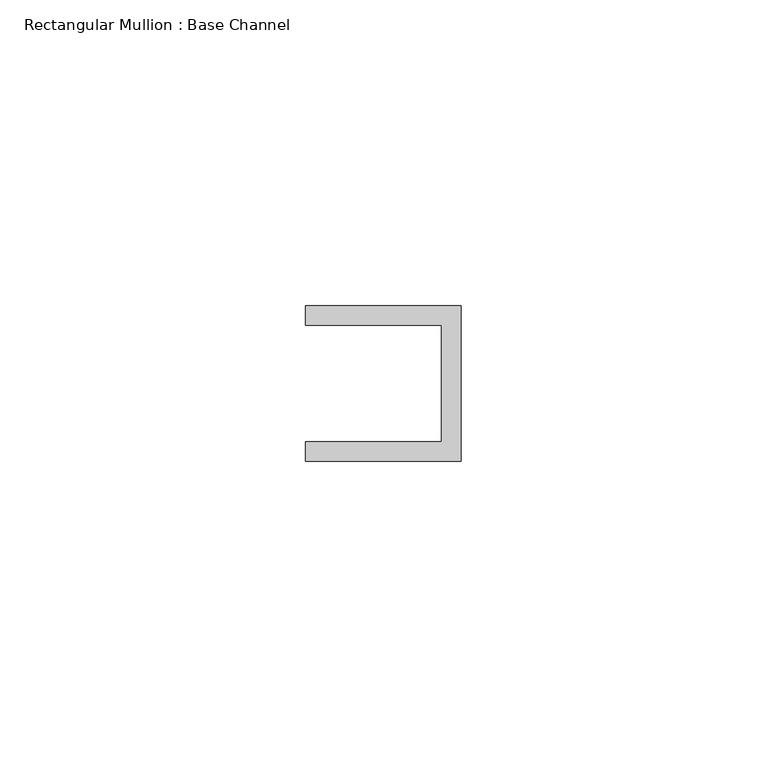
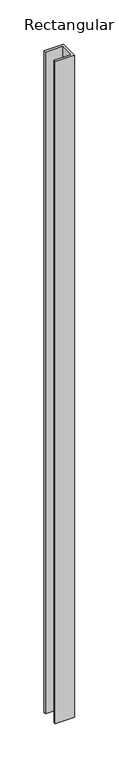
"""IFC4 building model written with IfcOpenShell, lengths in millimetres: member geometry, Rectangular Mullion : Base Channel."""

from ifc_helpers import new_model, si_unit, frame, origin, place, context, project, spatial, polyline, outline, extrude, source, transform, mapped, element, save


def rectangular_mullion_base_channel_70110dda(model_context):
    return source(origin(), model_context, "Body", "SweptSolid", [
        extrude(outline(polyline([(0.0, -12.7), (-25.4, -12.7), (-25.4, -9.525), (-3.175, -9.525), (-3.175, 9.525), (-25.4, 9.525), (-25.4, 12.7), (0.0, 12.7), (0.0, -12.7)])), frame((0.0, 0.0, -912.8125), z_axis=(0.0, 0.0, 1.0), x_axis=(1.0, 0.0, 0.0)), (0.0, 0.0, 1.0), 912.8125),
    ])


if __name__ == "__main__":
    model = new_model("IFC4")
    model_context = context("Model", 3, world=origin())
    ifc_project = project(units=[si_unit("LENGTHUNIT", "METRE", prefix="MILLI")], contexts=[model_context])
    site = spatial("IfcSite", under=ifc_project)
    building = spatial("IfcBuilding", under=site)
    placement = place(None, origin())
    rectangular_mullion_base_channel_shape = rectangular_mullion_base_channel_70110dda(model_context)
    element("IfcMember", 1, ObjectType="Rectangular Mullion : Base Channel", at=placement, inside=building, context=model_context, shape_type="MappedRepresentation", body=[
        mapped(rectangular_mullion_base_channel_shape, transform((0.0, 0.0, 0.0), x_axis=(1.0, 0.0, 0.0), y_axis=(0.0, 1.0, 0.0), z_axis=(0.0, 0.0, 1.0))),
    ])
    save(model, "model.ifc")

# Revit data of these elements
# Type "Rectangular Mullion : Base Channel"
#   built-in parameter 1007322 = 0.0833333 (stored number, unit not read)
#   built-in parameter 1007321 = 0.0416667 (stored number, unit not read)
#   built-in parameter 1007320 = -0.03125 (stored number, unit not read)
# Element 1 (IfcMember, "Rectangular Mullion : Base Channel")
#   Materials on its faces: "ALUM"
# Materials
#   "ALUM": class "Generic", colour RGB 157 157 157, transparency 0, Cost = 0
